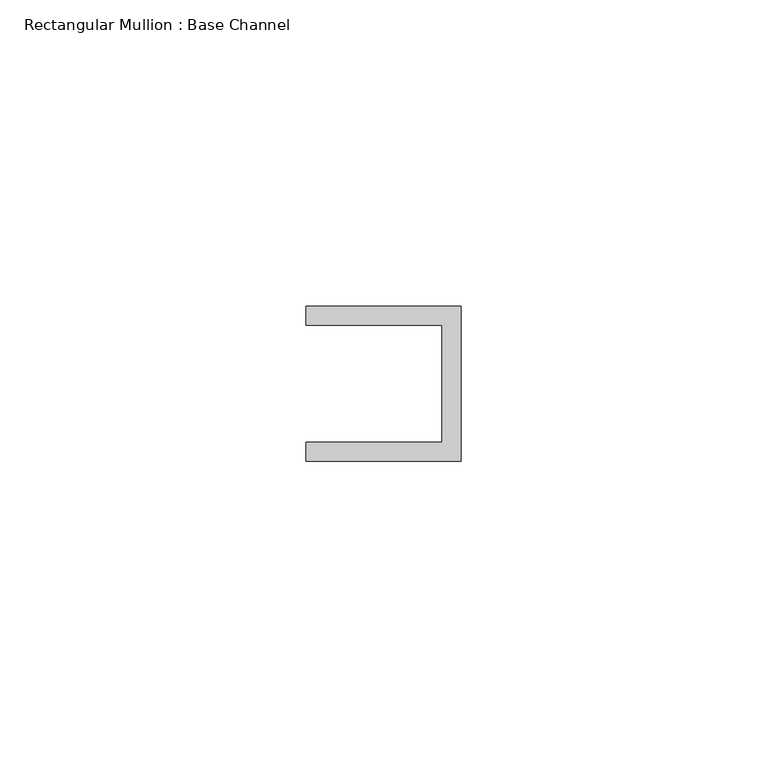
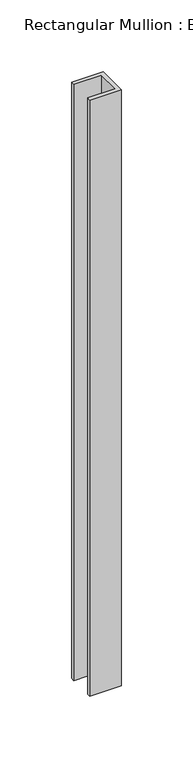
"""IFC4 building model written with IfcOpenShell, lengths in millimetres: member geometry, Rectangular Mullion : Base Channel."""

from ifc_helpers import new_model, si_unit, frame, origin, place, context, project, spatial, polyline, outline, extrude, source, transform, mapped, element, save


def rectangular_mullion_base_channel_3c473457(model_context):
    return source(origin(), model_context, "Body", "SweptSolid", [
        extrude(outline(polyline([(0.0, -12.7), (-25.4, -12.7), (-25.4, -9.525), (-3.175, -9.525), (-3.175, 9.525), (-25.4, 9.525), (-25.4, 12.7), (0.0, 12.7), (0.0, -12.7)])), frame((0.0, 0.0, -508.0), z_axis=(0.0, 0.0, 1.0), x_axis=(1.0, 0.0, 0.0)), (0.0, 0.0, 1.0), 508.0),
    ])


if __name__ == "__main__":
    model = new_model("IFC4")
    model_context = context("Model", 3, world=origin())
    ifc_project = project(units=[si_unit("LENGTHUNIT", "METRE", prefix="MILLI")], contexts=[model_context])
    site = spatial("IfcSite", under=ifc_project)
    building = spatial("IfcBuilding", under=site)
    placement = place(None, origin())
    rectangular_mullion_base_channel_shape = rectangular_mullion_base_channel_3c473457(model_context)
    element("IfcMember", 1, ObjectType="Rectangular Mullion : Base Channel", at=placement, inside=building, context=model_context, shape_type="MappedRepresentation", body=[
        mapped(rectangular_mullion_base_channel_shape, transform((0.0, 0.0, 0.0), x_axis=(1.0, 0.0, 0.0), y_axis=(0.0, 1.0, 0.0), z_axis=(0.0, 0.0, 1.0))),
    ])
    save(model, "model.ifc")

# Revit data of these elements
# Type "Rectangular Mullion : Base Channel"
#   built-in parameter 1007322 = 0.0833333 (stored number, unit not read)
#   built-in parameter 1007321 = 0.0416667 (stored number, unit not read)
#   built-in parameter 1007320 = -0.03125 (stored number, unit not read)
# Element 1 (IfcMember, "Rectangular Mullion : Base Channel")
#   Materials on its faces: "ALUM"
# Materials
#   "ALUM": class "Generic", colour RGB 157 157 157, transparency 0, Cost = 0
